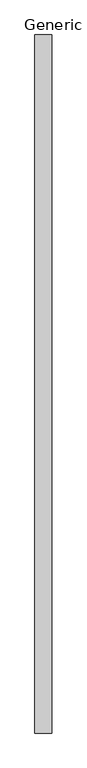
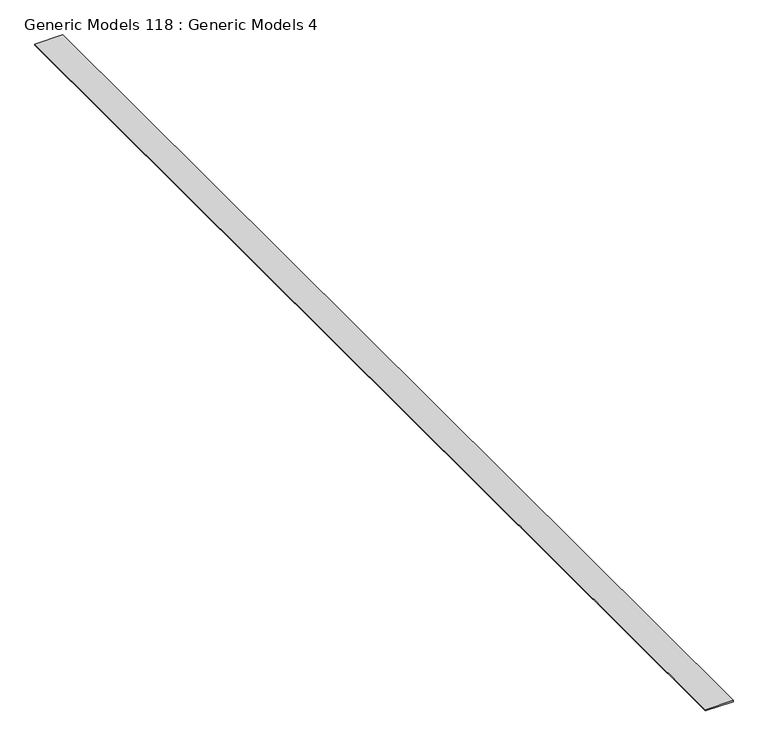
"""IFC4 building model written with IfcOpenShell, lengths in millimetres: proxy geometry, Generic Models 118 : Generic Models 4."""

from ifc_helpers import new_model, si_unit, frame, origin, place, context, project, spatial, polyline, outline, extrude, source, transform, mapped, element, save


def generic_models_118_generic_models_4_09d7919c(model_context):
    return source(origin(), model_context, "Body", "SweptSolid", [
        extrude(outline(polyline([(-6062.2158144, -6864.9230338), (-6508.088527, -6864.9230338), (-6508.088527, 11778.6769662), (-6062.2158144, 11778.6769662), (-6062.2158144, -6864.9230338)])), frame((0.0, 0.0, 126193.0878287), z_axis=(0.0, 0.0, 1.0), x_axis=(1.0, 0.0, 0.0)), (0.0, 0.0, 1.0), 18.3199747),
    ])


if __name__ == "__main__":
    model = new_model("IFC4")
    model_context = context("Model", 3, world=origin())
    ifc_project = project(units=[si_unit("LENGTHUNIT", "METRE", prefix="MILLI")], contexts=[model_context])
    site = spatial("IfcSite", under=ifc_project)
    building = spatial("IfcBuilding", under=site)
    placement = place(None, origin())
    generic_models_118_generic_models_4_shape = generic_models_118_generic_models_4_09d7919c(model_context)
    element("IfcBuildingElementProxy", 1, Name="Generic Models 118 : Generic Models 4", ObjectType="Generic Models 118 : Generic Models 4", at=placement, inside=building, context=model_context, shape_type="MappedRepresentation", body=[
        mapped(generic_models_118_generic_models_4_shape, transform((0.0, 0.0, 0.0), x_axis=(1.0, 0.0, 0.0), y_axis=(0.0, 1.0, 0.0), z_axis=(0.0, 0.0, 1.0))),
    ])
    save(model, "model.ifc")

# Revit data of these elements
# Element 1 (IfcBuildingElementProxy, "Generic Models 118 : Generic Models 4")
#   Materials on its faces: "_5/8\" DRYWALL"
# Materials
#   "_5/8\" DRYWALL": class "Generic", colour RGB 191 191 191, transparency 0, Cost = 0
